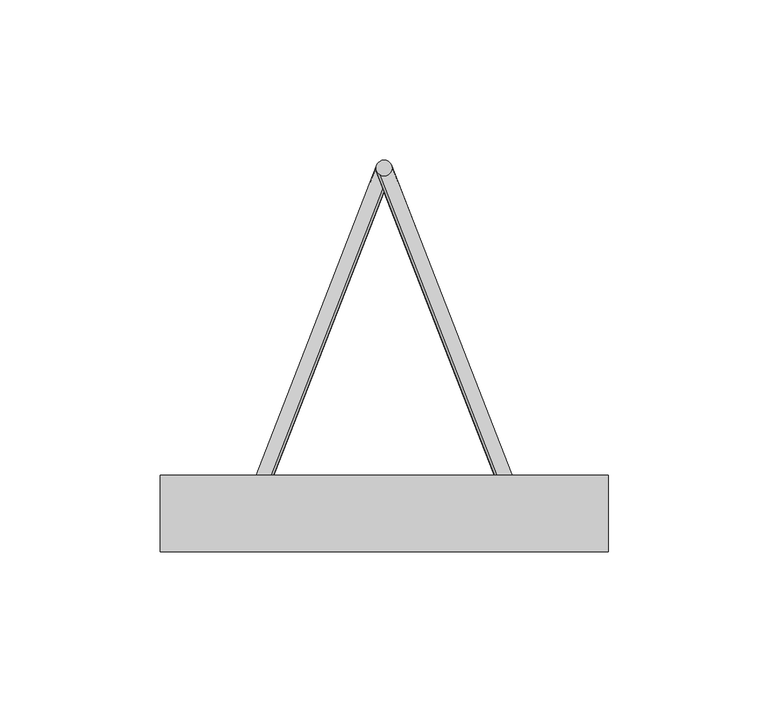
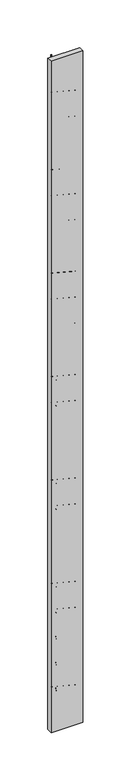
"""IFC4 building model written with IfcOpenShell, lengths in millimetres: proxy geometry, Vigota 7 (Pano 3) (Mf = 137)."""

from ifc_helpers import new_model, si_unit, point, frame, frame_2d, origin, origin_with_axes, origin_2d, place, context, project, spatial, polyline, circle_curve, trimmed, segment, composite_curve, outline, extrude, source, transform, mapped, element, save


def structural_framing_4e036d4d(model_context):
    return source(origin(), model_context, "Body", "SweptSolid", [
        extrude(outline(polyline([(-70.0, 12.0), (70.0, 12.0), (70.0, -12.0), (-70.0, -12.0), (-70.0, 12.0)])), origin_with_axes(), (0.0, 0.0, 1.0), 3115.00107),
        extrude(outline(composite_curve([segment(trimmed(circle_curve(frame_2d((42.0, 0.0)), 2.5), [point((44.5, 0.0))], [point((39.5, 0.0))], False, "CARTESIAN"), True, "CONTINUOUS"), segment(trimmed(circle_curve(frame_2d((42.0, 0.0)), 2.5), [point((39.5, 0.0))], [point((44.5, 0.0))], False, "CARTESIAN"), True, "CONTINUOUS")], self_intersect=False)), frame((0.0, 0.0, 28.0), z_axis=(0.0, 0.0, 1.0), x_axis=(1.0, 0.0, 0.0)), (0.0, 0.0, 1.0), 3059.00107),
        extrude(outline(composite_curve([segment(trimmed(circle_curve(frame_2d((0.0, 108.0)), 2.5), [point((2.5, 108.0))], [point((-2.5, 108.0))], False, "CARTESIAN"), True, "CONTINUOUS"), segment(trimmed(circle_curve(frame_2d((0.0, 108.0)), 2.5), [point((-2.5, 108.0))], [point((2.5, 108.0))], False, "CARTESIAN"), True, "CONTINUOUS")], self_intersect=False)), frame((0.0, 0.0, 67.500535), z_axis=(0.0, 0.0, 1.0), x_axis=(1.0, 0.0, 0.0)), (0.0, 0.0, 1.0), 2980.0),
        extrude(outline(composite_curve([segment(trimmed(circle_curve(origin_2d(), 2.5), [point((2.5, 0.0))], [point((-2.5, 0.0))], False, "CARTESIAN"), True, "CONTINUOUS"), segment(trimmed(circle_curve(origin_2d(), 2.5), [point((-2.5, 0.0))], [point((2.5, 0.0))], False, "CARTESIAN"), True, "CONTINUOUS")], self_intersect=False)), frame((42.0, 0.0, 57.500535), z_axis=(-0.3218603428886276, 0.8276408817707567, 0.4598004898837537), x_axis=(0.8192319205108605, -3.936835275445103e-11, 0.5734623443750141)), (0.0, 0.0, 1.0), 130.491379),
        extrude(outline(composite_curve([segment(trimmed(circle_curve(origin_2d(), 2.5), [point((2.5, 0.0))], [point((-2.5, 0.0))], False, "CARTESIAN"), True, "CONTINUOUS"), segment(trimmed(circle_curve(origin_2d(), 2.5), [point((-2.5, 0.0))], [point((2.5, 0.0))], False, "CARTESIAN"), True, "CONTINUOUS")], self_intersect=False)), frame((0.0, 108.0, 117.500535), z_axis=(0.3218603428886276, -0.8276408817707567, 0.4598004898837537), x_axis=(0.8192319205108605, -3.936835275445103e-11, -0.5734623443750141)), (0.0, 0.0, 1.0), 130.491379),
        extrude(outline(composite_curve([segment(trimmed(circle_curve(origin_2d(), 2.5), [point((2.5, 0.0))], [point((-2.5, 0.0))], False, "CARTESIAN"), True, "CONTINUOUS"), segment(trimmed(circle_curve(origin_2d(), 2.5), [point((-2.5, 0.0))], [point((2.5, 0.0))], False, "CARTESIAN"), True, "CONTINUOUS")], self_intersect=False)), frame((42.0, 0.0, 177.500535), z_axis=(-0.3218603428886276, 0.8276408817707567, 0.4598004898837537), x_axis=(0.8192319205108605, -3.936835275445103e-11, 0.5734623443750141)), (0.0, 0.0, 1.0), 130.491379),
        extrude(outline(composite_curve([segment(trimmed(circle_curve(origin_2d(), 2.5), [point((2.5, 0.0))], [point((-2.5, 0.0))], False, "CARTESIAN"), True, "CONTINUOUS"), segment(trimmed(circle_curve(origin_2d(), 2.5), [point((-2.5, 0.0))], [point((2.5, 0.0))], False, "CARTESIAN"), True, "CONTINUOUS")], self_intersect=False)), frame((0.0, 108.0, 237.500535), z_axis=(0.3218603428886276, -0.8276408817707567, 0.4598004898837537), x_axis=(0.8192319205108605, -3.936835275445103e-11, -0.5734623443750141)), (0.0, 0.0, 1.0), 130.491379),
        extrude(outline(composite_curve([segment(trimmed(circle_curve(origin_2d(), 2.5), [point((2.5, 0.0))], [point((-2.5, 0.0))], False, "CARTESIAN"), True, "CONTINUOUS"), segment(trimmed(circle_curve(origin_2d(), 2.5), [point((-2.5, 0.0))], [point((2.5, 0.0))], False, "CARTESIAN"), True, "CONTINUOUS")], self_intersect=False)), frame((42.0, 0.0, 297.500535), z_axis=(-0.3218603428886276, 0.8276408817707567, 0.4598004898837537), x_axis=(0.8192319205108605, -3.936835275445103e-11, 0.5734623443750141)), (0.0, 0.0, 1.0), 130.491379),
        extrude(outline(composite_curve([segment(trimmed(circle_curve(origin_2d(), 2.5), [point((2.5, 0.0))], [point((-2.5, 0.0))], False, "CARTESIAN"), True, "CONTINUOUS"), segment(trimmed(circle_curve(origin_2d(), 2.5), [point((-2.5, 0.0))], [point((2.5, 0.0))], False, "CARTESIAN"), True, "CONTINUOUS")], self_intersect=False)), frame((0.0, 108.0, 357.500535), z_axis=(0.3218603428886276, -0.8276408817707567, 0.4598004898837537), x_axis=(0.8192319205108605, -3.936835275445103e-11, -0.5734623443750141)), (0.0, 0.0, 1.0), 130.491379),
        extrude(outline(composite_curve([segment(trimmed(circle_curve(origin_2d(), 2.5), [point((2.5, 0.0))], [point((-2.5, 0.0))], False, "CARTESIAN"), True, "CONTINUOUS"), segment(trimmed(circle_curve(origin_2d(), 2.5), [point((-2.5, 0.0))], [point((2.5, 0.0))], False, "CARTESIAN"), True, "CONTINUOUS")], self_intersect=False)), frame((42.0, 0.0, 417.500535), z_axis=(-0.3218603428886276, 0.8276408817707567, 0.4598004898837537), x_axis=(0.8192319205108605, -3.936835275445103e-11, 0.5734623443750141)), (0.0, 0.0, 1.0), 130.491379),
        extrude(outline(composite_curve([segment(trimmed(circle_curve(origin_2d(), 2.5), [point((2.5, 0.0))], [point((-2.5, 0.0))], False, "CARTESIAN"), True, "CONTINUOUS"), segment(trimmed(circle_curve(origin_2d(), 2.5), [point((-2.5, 0.0))], [point((2.5, 0.0))], False, "CARTESIAN"), True, "CONTINUOUS")], self_intersect=False)), frame((0.0, 108.0, 477.500535), z_axis=(0.3218603428886276, -0.8276408817707567, 0.4598004898837537), x_axis=(0.8192319205108605, -3.936835275445103e-11, -0.5734623443750141)), (0.0, 0.0, 1.0), 130.491379),
        extrude(outline(composite_curve([segment(trimmed(circle_curve(origin_2d(), 2.5), [point((2.5, 0.0))], [point((-2.5, 0.0))], False, "CARTESIAN"), True, "CONTINUOUS"), segment(trimmed(circle_curve(origin_2d(), 2.5), [point((-2.5, 0.0))], [point((2.5, 0.0))], False, "CARTESIAN"), True, "CONTINUOUS")], self_intersect=False)), frame((42.0, 0.0, 537.500535), z_axis=(-0.3218603428886276, 0.8276408817707567, 0.4598004898837537), x_axis=(0.8192319205108605, -3.936835275445103e-11, 0.5734623443750141)), (0.0, 0.0, 1.0), 130.491379),
        extrude(outline(composite_curve([segment(trimmed(circle_curve(origin_2d(), 2.5), [point((2.5, 0.0))], [point((-2.5, 0.0))], False, "CARTESIAN"), True, "CONTINUOUS"), segment(trimmed(circle_curve(origin_2d(), 2.5), [point((-2.5, 0.0))], [point((2.5, 0.0))], False, "CARTESIAN"), True, "CONTINUOUS")], self_intersect=False)), frame((0.0, 108.0, 597.500535), z_axis=(0.3218603428886276, -0.8276408817707567, 0.4598004898837537), x_axis=(0.8192319205108605, -3.936835275445103e-11, -0.5734623443750141)), (0.0, 0.0, 1.0), 130.491379),
        extrude(outline(composite_curve([segment(trimmed(circle_curve(origin_2d(), 2.5), [point((2.5, 0.0))], [point((-2.5, 0.0))], False, "CARTESIAN"), True, "CONTINUOUS"), segment(trimmed(circle_curve(origin_2d(), 2.5), [point((-2.5, 0.0))], [point((2.5, 0.0))], False, "CARTESIAN"), True, "CONTINUOUS")], self_intersect=False)), frame((42.0, 0.0, 657.500535), z_axis=(-0.3218603428886276, 0.8276408817707567, 0.4598004898837537), x_axis=(0.8192319205108605, -3.936835275445103e-11, 0.5734623443750141)), (0.0, 0.0, 1.0), 130.491379),
        extrude(outline(composite_curve([segment(trimmed(circle_curve(origin_2d(), 2.5), [point((2.5, 0.0))], [point((-2.5, 0.0))], False, "CARTESIAN"), True, "CONTINUOUS"), segment(trimmed(circle_curve(origin_2d(), 2.5), [point((-2.5, 0.0))], [point((2.5, 0.0))], False, "CARTESIAN"), True, "CONTINUOUS")], self_intersect=False)), frame((0.0, 108.0, 717.500535), z_axis=(0.3218603428886276, -0.8276408817707567, 0.4598004898837537), x_axis=(0.8192319205108605, -3.936835275445103e-11, -0.5734623443750141)), (0.0, 0.0, 1.0), 130.491379),
        extrude(outline(composite_curve([segment(trimmed(circle_curve(origin_2d(), 2.5), [point((2.5, 0.0))], [point((-2.5, 0.0))], False, "CARTESIAN"), True, "CONTINUOUS"), segment(trimmed(circle_curve(origin_2d(), 2.5), [point((-2.5, 0.0))], [point((2.5, 0.0))], False, "CARTESIAN"), True, "CONTINUOUS")], self_intersect=False)), frame((42.0, 0.0, 777.500535), z_axis=(-0.3218603428886276, 0.8276408817707567, 0.4598004898837537), x_axis=(0.8192319205108605, -3.936835275445103e-11, 0.5734623443750141)), (0.0, 0.0, 1.0), 130.491379),
        extrude(outline(composite_curve([segment(trimmed(circle_curve(origin_2d(), 2.5), [point((2.5, 0.0))], [point((-2.5, 0.0))], False, "CARTESIAN"), True, "CONTINUOUS"), segment(trimmed(circle_curve(origin_2d(), 2.5), [point((-2.5, 0.0))], [point((2.5, 0.0))], False, "CARTESIAN"), True, "CONTINUOUS")], self_intersect=False)), frame((0.0, 108.0, 837.500535), z_axis=(0.3218603428886276, -0.8276408817707567, 0.4598004898837537), x_axis=(0.8192319205108605, -3.936835275445103e-11, -0.5734623443750141)), (0.0, 0.0, 1.0), 130.491379),
        extrude(outline(composite_curve([segment(trimmed(circle_curve(origin_2d(), 2.5), [point((2.5, 0.0))], [point((-2.5, 0.0))], False, "CARTESIAN"), True, "CONTINUOUS"), segment(trimmed(circle_curve(origin_2d(), 2.5), [point((-2.5, 0.0))], [point((2.5, 0.0))], False, "CARTESIAN"), True, "CONTINUOUS")], self_intersect=False)), frame((42.0, 0.0, 897.500535), z_axis=(-0.3218603428886276, 0.8276408817707567, 0.4598004898837537), x_axis=(0.8192319205108605, -3.936835275445103e-11, 0.5734623443750141)), (0.0, 0.0, 1.0), 130.491379),
        extrude(outline(composite_curve([segment(trimmed(circle_curve(origin_2d(), 2.5), [point((2.5, 0.0))], [point((-2.5, 0.0))], False, "CARTESIAN"), True, "CONTINUOUS"), segment(trimmed(circle_curve(origin_2d(), 2.5), [point((-2.5, 0.0))], [point((2.5, 0.0))], False, "CARTESIAN"), True, "CONTINUOUS")], self_intersect=False)), frame((0.0, 108.0, 957.500535), z_axis=(0.3218603428886276, -0.8276408817707567, 0.4598004898837537), x_axis=(0.8192319205108605, -3.936835275445103e-11, -0.5734623443750141)), (0.0, 0.0, 1.0), 130.491379),
        extrude(outline(composite_curve([segment(trimmed(circle_curve(origin_2d(), 2.5), [point((2.5, 0.0))], [point((-2.5, 0.0))], False, "CARTESIAN"), True, "CONTINUOUS"), segment(trimmed(circle_curve(origin_2d(), 2.5), [point((-2.5, 0.0))], [point((2.5, 0.0))], False, "CARTESIAN"), True, "CONTINUOUS")], self_intersect=False)), frame((42.0, 0.0, 1017.500535), z_axis=(-0.3218603428886276, 0.8276408817707567, 0.4598004898837537), x_axis=(0.8192319205108605, -3.936835275445103e-11, 0.5734623443750141)), (0.0, 0.0, 1.0), 130.491379),
        extrude(outline(composite_curve([segment(trimmed(circle_curve(origin_2d(), 2.5), [point((2.5, 0.0))], [point((-2.5, 0.0))], False, "CARTESIAN"), True, "CONTINUOUS"), segment(trimmed(circle_curve(origin_2d(), 2.5), [point((-2.5, 0.0))], [point((2.5, 0.0))], False, "CARTESIAN"), True, "CONTINUOUS")], self_intersect=False)), frame((0.0, 108.0, 1077.500535), z_axis=(0.3218603428886276, -0.8276408817707567, 0.4598004898837537), x_axis=(0.8192319205108605, -3.936835275445103e-11, -0.5734623443750141)), (0.0, 0.0, 1.0), 130.491379),
        extrude(outline(composite_curve([segment(trimmed(circle_curve(origin_2d(), 2.5), [point((2.5, 0.0))], [point((-2.5, 0.0))], False, "CARTESIAN"), True, "CONTINUOUS"), segment(trimmed(circle_curve(origin_2d(), 2.5), [point((-2.5, 0.0))], [point((2.5, 0.0))], False, "CARTESIAN"), True, "CONTINUOUS")], self_intersect=False)), frame((42.0, 0.0, 1137.500535), z_axis=(-0.3218603428886276, 0.8276408817707567, 0.4598004898837537), x_axis=(0.8192319205108605, -3.936835275445103e-11, 0.5734623443750141)), (0.0, 0.0, 1.0), 130.491379),
        extrude(outline(composite_curve([segment(trimmed(circle_curve(origin_2d(), 2.5), [point((2.5, 0.0))], [point((-2.5, 0.0))], False, "CARTESIAN"), True, "CONTINUOUS"), segment(trimmed(circle_curve(origin_2d(), 2.5), [point((-2.5, 0.0))], [point((2.5, 0.0))], False, "CARTESIAN"), True, "CONTINUOUS")], self_intersect=False)), frame((0.0, 108.0, 1197.500535), z_axis=(0.3218603428886276, -0.8276408817707567, 0.4598004898837537), x_axis=(0.8192319205108605, -3.936835275445103e-11, -0.5734623443750141)), (0.0, 0.0, 1.0), 130.491379),
        extrude(outline(composite_curve([segment(trimmed(circle_curve(origin_2d(), 2.5), [point((2.5, 0.0))], [point((-2.5, 0.0))], False, "CARTESIAN"), True, "CONTINUOUS"), segment(trimmed(circle_curve(origin_2d(), 2.5), [point((-2.5, 0.0))], [point((2.5, 0.0))], False, "CARTESIAN"), True, "CONTINUOUS")], self_intersect=False)), frame((42.0, 0.0, 1257.500535), z_axis=(-0.3218603428886276, 0.8276408817707567, 0.4598004898837537), x_axis=(0.8192319205108605, -3.936835275445103e-11, 0.5734623443750141)), (0.0, 0.0, 1.0), 130.491379),
        extrude(outline(composite_curve([segment(trimmed(circle_curve(origin_2d(), 2.5), [point((2.5, 0.0))], [point((-2.5, 0.0))], False, "CARTESIAN"), True, "CONTINUOUS"), segment(trimmed(circle_curve(origin_2d(), 2.5), [point((-2.5, 0.0))], [point((2.5, 0.0))], False, "CARTESIAN"), True, "CONTINUOUS")], self_intersect=False)), frame((0.0, 108.0, 1317.500535), z_axis=(0.3218603428886276, -0.8276408817707567, 0.4598004898837537), x_axis=(0.8192319205108605, -3.936835275445103e-11, -0.5734623443750141)), (0.0, 0.0, 1.0), 130.491379),
        extrude(outline(composite_curve([segment(trimmed(circle_curve(origin_2d(), 2.5), [point((2.5, 0.0))], [point((-2.5, 0.0))], False, "CARTESIAN"), True, "CONTINUOUS"), segment(trimmed(circle_curve(origin_2d(), 2.5), [point((-2.5, 0.0))], [point((2.5, 0.0))], False, "CARTESIAN"), True, "CONTINUOUS")], self_intersect=False)), frame((42.0, 0.0, 1377.500535), z_axis=(-0.3218603428886276, 0.8276408817707567, 0.4598004898837537), x_axis=(0.8192319205108605, -3.936835275445103e-11, 0.5734623443750141)), (0.0, 0.0, 1.0), 130.491379),
        extrude(outline(composite_curve([segment(trimmed(circle_curve(origin_2d(), 2.5), [point((2.5, 0.0))], [point((-2.5, 0.0))], False, "CARTESIAN"), True, "CONTINUOUS"), segment(trimmed(circle_curve(origin_2d(), 2.5), [point((-2.5, 0.0))], [point((2.5, 0.0))], False, "CARTESIAN"), True, "CONTINUOUS")], self_intersect=False)), frame((0.0, 108.0, 1437.500535), z_axis=(0.3218603428886276, -0.8276408817707567, 0.4598004898837537), x_axis=(0.8192319205108605, -3.936835275445103e-11, -0.5734623443750141)), (0.0, 0.0, 1.0), 130.491379),
        extrude(outline(composite_curve([segment(trimmed(circle_curve(origin_2d(), 2.5), [point((2.5, 0.0))], [point((-2.5, 0.0))], False, "CARTESIAN"), True, "CONTINUOUS"), segment(trimmed(circle_curve(origin_2d(), 2.5), [point((-2.5, 0.0))], [point((2.5, 0.0))], False, "CARTESIAN"), True, "CONTINUOUS")], self_intersect=False)), frame((42.0, 0.0, 1497.500535), z_axis=(-0.3218603428886276, 0.8276408817707567, 0.4598004898837537), x_axis=(0.8192319205108605, -3.936835275445103e-11, 0.5734623443750141)), (0.0, 0.0, 1.0), 130.491379),
        extrude(outline(composite_curve([segment(trimmed(circle_curve(origin_2d(), 2.5), [point((2.5, 0.0))], [point((-2.5, 0.0))], False, "CARTESIAN"), True, "CONTINUOUS"), segment(trimmed(circle_curve(origin_2d(), 2.5), [point((-2.5, 0.0))], [point((2.5, 0.0))], False, "CARTESIAN"), True, "CONTINUOUS")], self_intersect=False)), frame((0.0, 108.0, 1557.500535), z_axis=(0.3218603428886276, -0.8276408817707567, 0.4598004898837537), x_axis=(0.8192319205108605, -3.936835275445103e-11, -0.5734623443750141)), (0.0, 0.0, 1.0), 130.491379),
        extrude(outline(composite_curve([segment(trimmed(circle_curve(origin_2d(), 2.5), [point((2.5, 0.0))], [point((-2.5, 0.0))], False, "CARTESIAN"), True, "CONTINUOUS"), segment(trimmed(circle_curve(origin_2d(), 2.5), [point((-2.5, 0.0))], [point((2.5, 0.0))], False, "CARTESIAN"), True, "CONTINUOUS")], self_intersect=False)), frame((42.0, 0.0, 1617.500535), z_axis=(-0.3218603428886276, 0.8276408817707567, 0.4598004898837537), x_axis=(0.8192319205108605, -3.936835275445103e-11, 0.5734623443750141)), (0.0, 0.0, 1.0), 130.491379),
        extrude(outline(composite_curve([segment(trimmed(circle_curve(origin_2d(), 2.5), [point((2.5, 0.0))], [point((-2.5, 0.0))], False, "CARTESIAN"), True, "CONTINUOUS"), segment(trimmed(circle_curve(origin_2d(), 2.5), [point((-2.5, 0.0))], [point((2.5, 0.0))], False, "CARTESIAN"), True, "CONTINUOUS")], self_intersect=False)), frame((0.0, 108.0, 1677.500535), z_axis=(0.3218603428886276, -0.8276408817707567, 0.4598004898837537), x_axis=(0.8192319205108605, -3.936835275445103e-11, -0.5734623443750141)), (0.0, 0.0, 1.0), 130.491379),
        extrude(outline(composite_curve([segment(trimmed(circle_curve(origin_2d(), 2.5), [point((2.5, 0.0))], [point((-2.5, 0.0))], False, "CARTESIAN"), True, "CONTINUOUS"), segment(trimmed(circle_curve(origin_2d(), 2.5), [point((-2.5, 0.0))], [point((2.5, 0.0))], False, "CARTESIAN"), True, "CONTINUOUS")], self_intersect=False)), frame((42.0, 0.0, 1737.500535), z_axis=(-0.3218603428886276, 0.8276408817707567, 0.4598004898837537), x_axis=(0.8192319205108605, -3.936835275445103e-11, 0.5734623443750141)), (0.0, 0.0, 1.0), 130.491379),
        extrude(outline(composite_curve([segment(trimmed(circle_curve(origin_2d(), 2.5), [point((2.5, 0.0))], [point((-2.5, 0.0))], False, "CARTESIAN"), True, "CONTINUOUS"), segment(trimmed(circle_curve(origin_2d(), 2.5), [point((-2.5, 0.0))], [point((2.5, 0.0))], False, "CARTESIAN"), True, "CONTINUOUS")], self_intersect=False)), frame((0.0, 108.0, 1797.500535), z_axis=(0.3218603428886276, -0.8276408817707567, 0.4598004898837537), x_axis=(0.8192319205108605, -3.936835275445103e-11, -0.5734623443750141)), (0.0, 0.0, 1.0), 130.491379),
        extrude(outline(composite_curve([segment(trimmed(circle_curve(origin_2d(), 2.5), [point((2.5, 0.0))], [point((-2.5, 0.0))], False, "CARTESIAN"), True, "CONTINUOUS"), segment(trimmed(circle_curve(origin_2d(), 2.5), [point((-2.5, 0.0))], [point((2.5, 0.0))], False, "CARTESIAN"), True, "CONTINUOUS")], self_intersect=False)), frame((42.0, 0.0, 1857.500535), z_axis=(-0.3218603428886276, 0.8276408817707567, 0.4598004898837537), x_axis=(0.8192319205108605, -3.936835275445103e-11, 0.5734623443750141)), (0.0, 0.0, 1.0), 130.491379),
        extrude(outline(composite_curve([segment(trimmed(circle_curve(origin_2d(), 2.5), [point((2.5, 0.0))], [point((-2.5, 0.0))], False, "CARTESIAN"), True, "CONTINUOUS"), segment(trimmed(circle_curve(origin_2d(), 2.5), [point((-2.5, 0.0))], [point((2.5, 0.0))], False, "CARTESIAN"), True, "CONTINUOUS")], self_intersect=False)), frame((0.0, 108.0, 1917.500535), z_axis=(0.3218603428886276, -0.8276408817707567, 0.4598004898837537), x_axis=(0.8192319205108605, -3.936835275445103e-11, -0.5734623443750141)), (0.0, 0.0, 1.0), 130.491379),
        extrude(outline(composite_curve([segment(trimmed(circle_curve(origin_2d(), 2.5), [point((2.5, 0.0))], [point((-2.5, 0.0))], False, "CARTESIAN"), True, "CONTINUOUS"), segment(trimmed(circle_curve(origin_2d(), 2.5), [point((-2.5, 0.0))], [point((2.5, 0.0))], False, "CARTESIAN"), True, "CONTINUOUS")], self_intersect=False)), frame((42.0, 0.0, 1977.500535), z_axis=(-0.3218603428886276, 0.8276408817707567, 0.4598004898837537), x_axis=(0.8192319205108605, -3.936835275445103e-11, 0.5734623443750141)), (0.0, 0.0, 1.0), 130.491379),
        extrude(outline(composite_curve([segment(trimmed(circle_curve(origin_2d(), 2.5), [point((2.5, 0.0))], [point((-2.5, 0.0))], False, "CARTESIAN"), True, "CONTINUOUS"), segment(trimmed(circle_curve(origin_2d(), 2.5), [point((-2.5, 0.0))], [point((2.5, 0.0))], False, "CARTESIAN"), True, "CONTINUOUS")], self_intersect=False)), frame((0.0, 108.0, 2037.500535), z_axis=(0.3218603428886276, -0.8276408817707567, 0.4598004898837537), x_axis=(0.8192319205108605, -3.936835275445103e-11, -0.5734623443750141)), (0.0, 0.0, 1.0), 130.491379),
        extrude(outline(composite_curve([segment(trimmed(circle_curve(origin_2d(), 2.5), [point((2.5, 0.0))], [point((-2.5, 0.0))], False, "CARTESIAN"), True, "CONTINUOUS"), segment(trimmed(circle_curve(origin_2d(), 2.5), [point((-2.5, 0.0))], [point((2.5, 0.0))], False, "CARTESIAN"), True, "CONTINUOUS")], self_intersect=False)), frame((42.0, 0.0, 2097.500535), z_axis=(-0.3218603428886276, 0.8276408817707567, 0.4598004898837537), x_axis=(0.8192319205108605, -3.936835275445103e-11, 0.5734623443750141)), (0.0, 0.0, 1.0), 130.491379),
        extrude(outline(composite_curve([segment(trimmed(circle_curve(origin_2d(), 2.5), [point((2.5, 0.0))], [point((-2.5, 0.0))], False, "CARTESIAN"), True, "CONTINUOUS"), segment(trimmed(circle_curve(origin_2d(), 2.5), [point((-2.5, 0.0))], [point((2.5, 0.0))], False, "CARTESIAN"), True, "CONTINUOUS")], self_intersect=False)), frame((0.0, 108.0, 2157.500535), z_axis=(0.3218603428886276, -0.8276408817707567, 0.4598004898837537), x_axis=(0.8192319205108605, -3.936835275445103e-11, -0.5734623443750141)), (0.0, 0.0, 1.0), 130.491379),
        extrude(outline(composite_curve([segment(trimmed(circle_curve(origin_2d(), 2.5), [point((2.5, 0.0))], [point((-2.5, 0.0))], False, "CARTESIAN"), True, "CONTINUOUS"), segment(trimmed(circle_curve(origin_2d(), 2.5), [point((-2.5, 0.0))], [point((2.5, 0.0))], False, "CARTESIAN"), True, "CONTINUOUS")], self_intersect=False)), frame((42.0, 0.0, 2217.500535), z_axis=(-0.3218603428886276, 0.8276408817707567, 0.4598004898837537), x_axis=(0.8192319205108605, -3.936835275445103e-11, 0.5734623443750141)), (0.0, 0.0, 1.0), 130.491379),
        extrude(outline(composite_curve([segment(trimmed(circle_curve(origin_2d(), 2.5), [point((2.5, 0.0))], [point((-2.5, 0.0))], False, "CARTESIAN"), True, "CONTINUOUS"), segment(trimmed(circle_curve(origin_2d(), 2.5), [point((-2.5, 0.0))], [point((2.5, 0.0))], False, "CARTESIAN"), True, "CONTINUOUS")], self_intersect=False)), frame((0.0, 108.0, 2277.500535), z_axis=(0.3218603428886276, -0.8276408817707567, 0.4598004898837537), x_axis=(0.8192319205108605, -3.936835275445103e-11, -0.5734623443750141)), (0.0, 0.0, 1.0), 130.491379),
        extrude(outline(composite_curve([segment(trimmed(circle_curve(origin_2d(), 2.5), [point((2.5, 0.0))], [point((-2.5, 0.0))], False, "CARTESIAN"), True, "CONTINUOUS"), segment(trimmed(circle_curve(origin_2d(), 2.5), [point((-2.5, 0.0))], [point((2.5, 0.0))], False, "CARTESIAN"), True, "CONTINUOUS")], self_intersect=False)), frame((42.0, 0.0, 2337.500535), z_axis=(-0.3218603428886276, 0.8276408817707567, 0.4598004898837537), x_axis=(0.8192319205108605, -3.936835275445103e-11, 0.5734623443750141)), (0.0, 0.0, 1.0), 130.491379),
        extrude(outline(composite_curve([segment(trimmed(circle_curve(origin_2d(), 2.5), [point((2.5, 0.0))], [point((-2.5, 0.0))], False, "CARTESIAN"), True, "CONTINUOUS"), segment(trimmed(circle_curve(origin_2d(), 2.5), [point((-2.5, 0.0))], [point((2.5, 0.0))], False, "CARTESIAN"), True, "CONTINUOUS")], self_intersect=False)), frame((0.0, 108.0, 2397.500535), z_axis=(0.3218603428886276, -0.8276408817707567, 0.4598004898837537), x_axis=(0.8192319205108605, -3.936835275445103e-11, -0.5734623443750141)), (0.0, 0.0, 1.0), 130.491379),
        extrude(outline(composite_curve([segment(trimmed(circle_curve(origin_2d(), 2.5), [point((2.5, 0.0))], [point((-2.5, 0.0))], False, "CARTESIAN"), True, "CONTINUOUS"), segment(trimmed(circle_curve(origin_2d(), 2.5), [point((-2.5, 0.0))], [point((2.5, 0.0))], False, "CARTESIAN"), True, "CONTINUOUS")], self_intersect=False)), frame((42.0, 0.0, 2457.500535), z_axis=(-0.3218603428886276, 0.8276408817707567, 0.4598004898837537), x_axis=(0.8192319205108605, -3.936835275445103e-11, 0.5734623443750141)), (0.0, 0.0, 1.0), 130.491379),
        extrude(outline(composite_curve([segment(trimmed(circle_curve(origin_2d(), 2.5), [point((2.5, 0.0))], [point((-2.5, 0.0))], False, "CARTESIAN"), True, "CONTINUOUS"), segment(trimmed(circle_curve(origin_2d(), 2.5), [point((-2.5, 0.0))], [point((2.5, 0.0))], False, "CARTESIAN"), True, "CONTINUOUS")], self_intersect=False)), frame((0.0, 108.0, 2517.500535), z_axis=(0.3218603428886276, -0.8276408817707567, 0.4598004898837537), x_axis=(0.8192319205108605, -3.936835275445103e-11, -0.5734623443750141)), (0.0, 0.0, 1.0), 130.491379),
        extrude(outline(composite_curve([segment(trimmed(circle_curve(origin_2d(), 2.5), [point((2.5, 0.0))], [point((-2.5, 0.0))], False, "CARTESIAN"), True, "CONTINUOUS"), segment(trimmed(circle_curve(origin_2d(), 2.5), [point((-2.5, 0.0))], [point((2.5, 0.0))], False, "CARTESIAN"), True, "CONTINUOUS")], self_intersect=False)), frame((42.0, 0.0, 2577.500535), z_axis=(-0.3218603428886276, 0.8276408817707567, 0.4598004898837537), x_axis=(0.8192319205108605, -3.936835275445103e-11, 0.5734623443750141)), (0.0, 0.0, 1.0), 130.491379),
        extrude(outline(composite_curve([segment(trimmed(circle_curve(origin_2d(), 2.5), [point((2.5, 0.0))], [point((-2.5, 0.0))], False, "CARTESIAN"), True, "CONTINUOUS"), segment(trimmed(circle_curve(origin_2d(), 2.5), [point((-2.5, 0.0))], [point((2.5, 0.0))], False, "CARTESIAN"), True, "CONTINUOUS")], self_intersect=False)), frame((0.0, 108.0, 2637.500535), z_axis=(0.3218603428886276, -0.8276408817707567, 0.4598004898837537), x_axis=(0.8192319205108605, -3.936835275445103e-11, -0.5734623443750141)), (0.0, 0.0, 1.0), 130.491379),
        extrude(outline(composite_curve([segment(trimmed(circle_curve(origin_2d(), 2.5), [point((2.5, 0.0))], [point((-2.5, 0.0))], False, "CARTESIAN"), True, "CONTINUOUS"), segment(trimmed(circle_curve(origin_2d(), 2.5), [point((-2.5, 0.0))], [point((2.5, 0.0))], False, "CARTESIAN"), True, "CONTINUOUS")], self_intersect=False)), frame((42.0, 0.0, 2697.500535), z_axis=(-0.3218603428886276, 0.8276408817707567, 0.4598004898837537), x_axis=(0.8192319205108605, -3.936835275445103e-11, 0.5734623443750141)), (0.0, 0.0, 1.0), 130.491379),
        extrude(outline(composite_curve([segment(trimmed(circle_curve(origin_2d(), 2.5), [point((2.5, 0.0))], [point((-2.5, 0.0))], False, "CARTESIAN"), True, "CONTINUOUS"), segment(trimmed(circle_curve(origin_2d(), 2.5), [point((-2.5, 0.0))], [point((2.5, 0.0))], False, "CARTESIAN"), True, "CONTINUOUS")], self_intersect=False)), frame((0.0, 108.0, 2757.500535), z_axis=(0.3218603428886276, -0.8276408817707567, 0.4598004898837537), x_axis=(0.8192319205108605, -3.936835275445103e-11, -0.5734623443750141)), (0.0, 0.0, 1.0), 130.491379),
        extrude(outline(composite_curve([segment(trimmed(circle_curve(origin_2d(), 2.5), [point((2.5, 0.0))], [point((-2.5, 0.0))], False, "CARTESIAN"), True, "CONTINUOUS"), segment(trimmed(circle_curve(origin_2d(), 2.5), [point((-2.5, 0.0))], [point((2.5, 0.0))], False, "CARTESIAN"), True, "CONTINUOUS")], self_intersect=False)), frame((42.0, 0.0, 2817.500535), z_axis=(-0.3218603428886276, 0.8276408817707567, 0.4598004898837537), x_axis=(0.8192319205108605, -3.936835275445103e-11, 0.5734623443750141)), (0.0, 0.0, 1.0), 130.491379),
        extrude(outline(composite_curve([segment(trimmed(circle_curve(origin_2d(), 2.5), [point((2.5, 0.0))], [point((-2.5, 0.0))], False, "CARTESIAN"), True, "CONTINUOUS"), segment(trimmed(circle_curve(origin_2d(), 2.5), [point((-2.5, 0.0))], [point((2.5, 0.0))], False, "CARTESIAN"), True, "CONTINUOUS")], self_intersect=False)), frame((0.0, 108.0, 2877.500535), z_axis=(0.3218603428886276, -0.8276408817707567, 0.4598004898837537), x_axis=(0.8192319205108605, -3.936835275445103e-11, -0.5734623443750141)), (0.0, 0.0, 1.0), 130.491379),
        extrude(outline(composite_curve([segment(trimmed(circle_curve(origin_2d(), 2.5), [point((2.5, 0.0))], [point((-2.5, 0.0))], False, "CARTESIAN"), True, "CONTINUOUS"), segment(trimmed(circle_curve(origin_2d(), 2.5), [point((-2.5, 0.0))], [point((2.5, 0.0))], False, "CARTESIAN"), True, "CONTINUOUS")], self_intersect=False)), frame((42.0, 0.0, 2937.500535), z_axis=(-0.3218603428886276, 0.8276408817707567, 0.4598004898837537), x_axis=(0.8192319205108605, -3.936835275445103e-11, 0.5734623443750141)), (0.0, 0.0, 1.0), 130.491379),
        extrude(outline(composite_curve([segment(trimmed(circle_curve(origin_2d(), 2.5), [point((2.5, 0.0))], [point((-2.5, 0.0))], False, "CARTESIAN"), True, "CONTINUOUS"), segment(trimmed(circle_curve(origin_2d(), 2.5), [point((-2.5, 0.0))], [point((2.5, 0.0))], False, "CARTESIAN"), True, "CONTINUOUS")], self_intersect=False)), frame((0.0, 108.0, 2997.500535), z_axis=(0.3218603428886276, -0.8276408817707567, 0.4598004898837537), x_axis=(0.8192319205108605, -3.936835275445103e-11, -0.5734623443750141)), (0.0, 0.0, 1.0), 130.491379),
        extrude(outline(composite_curve([segment(trimmed(circle_curve(frame_2d((-42.0, 0.0)), 2.5), [point((-39.5, 0.0))], [point((-44.5, 0.0))], False, "CARTESIAN"), True, "CONTINUOUS"), segment(trimmed(circle_curve(frame_2d((-42.0, 0.0)), 2.5), [point((-44.5, 0.0))], [point((-39.5, 0.0))], False, "CARTESIAN"), True, "CONTINUOUS")], self_intersect=False)), frame((0.0, 0.0, 28.0), z_axis=(0.0, 0.0, 1.0), x_axis=(1.0, 0.0, 0.0)), (0.0, 0.0, 1.0), 3059.00107),
        extrude(outline(composite_curve([segment(trimmed(circle_curve(origin_2d(), 2.5), [point((2.5, 0.0))], [point((-2.5, 0.0))], False, "CARTESIAN"), True, "CONTINUOUS"), segment(trimmed(circle_curve(origin_2d(), 2.5), [point((-2.5, 0.0))], [point((2.5, 0.0))], False, "CARTESIAN"), True, "CONTINUOUS")], self_intersect=False)), frame((-42.0, 0.0, 57.500535), z_axis=(0.3218603428886276, 0.8276408817707567, 0.4598004898837537), x_axis=(0.8192319205108605, 3.936835275445103e-11, -0.5734623443750141)), (0.0, 0.0, 1.0), 130.491379),
        extrude(outline(composite_curve([segment(trimmed(circle_curve(origin_2d(), 2.5), [point((2.5, 0.0))], [point((-2.5, 0.0))], False, "CARTESIAN"), True, "CONTINUOUS"), segment(trimmed(circle_curve(origin_2d(), 2.5), [point((-2.5, 0.0))], [point((2.5, 0.0))], False, "CARTESIAN"), True, "CONTINUOUS")], self_intersect=False)), frame((0.0, 108.0, 117.500535), z_axis=(-0.3218603428886276, -0.8276408817707567, 0.4598004898837537), x_axis=(0.8192319205108605, 3.936835275445103e-11, 0.5734623443750141)), (0.0, 0.0, 1.0), 130.491379),
        extrude(outline(composite_curve([segment(trimmed(circle_curve(origin_2d(), 2.5), [point((2.5, 0.0))], [point((-2.5, 0.0))], False, "CARTESIAN"), True, "CONTINUOUS"), segment(trimmed(circle_curve(origin_2d(), 2.5), [point((-2.5, 0.0))], [point((2.5, 0.0))], False, "CARTESIAN"), True, "CONTINUOUS")], self_intersect=False)), frame((-42.0, 0.0, 177.500535), z_axis=(0.3218603428886276, 0.8276408817707567, 0.4598004898837537), x_axis=(0.8192319205108605, 3.936835275445103e-11, -0.5734623443750141)), (0.0, 0.0, 1.0), 130.491379),
        extrude(outline(composite_curve([segment(trimmed(circle_curve(origin_2d(), 2.5), [point((2.5, 0.0))], [point((-2.5, 0.0))], False, "CARTESIAN"), True, "CONTINUOUS"), segment(trimmed(circle_curve(origin_2d(), 2.5), [point((-2.5, 0.0))], [point((2.5, 0.0))], False, "CARTESIAN"), True, "CONTINUOUS")], self_intersect=False)), frame((0.0, 108.0, 237.500535), z_axis=(-0.3218603428886276, -0.8276408817707567, 0.4598004898837537), x_axis=(0.8192319205108605, 3.936835275445103e-11, 0.5734623443750141)), (0.0, 0.0, 1.0), 130.491379),
        extrude(outline(composite_curve([segment(trimmed(circle_curve(origin_2d(), 2.5), [point((2.5, 0.0))], [point((-2.5, 0.0))], False, "CARTESIAN"), True, "CONTINUOUS"), segment(trimmed(circle_curve(origin_2d(), 2.5), [point((-2.5, 0.0))], [point((2.5, 0.0))], False, "CARTESIAN"), True, "CONTINUOUS")], self_intersect=False)), frame((-42.0, 0.0, 297.500535), z_axis=(0.3218603428886276, 0.8276408817707567, 0.4598004898837537), x_axis=(0.8192319205108605, 3.936835275445103e-11, -0.5734623443750141)), (0.0, 0.0, 1.0), 130.491379),
        extrude(outline(composite_curve([segment(trimmed(circle_curve(origin_2d(), 2.5), [point((2.5, 0.0))], [point((-2.5, 0.0))], False, "CARTESIAN"), True, "CONTINUOUS"), segment(trimmed(circle_curve(origin_2d(), 2.5), [point((-2.5, 0.0))], [point((2.5, 0.0))], False, "CARTESIAN"), True, "CONTINUOUS")], self_intersect=False)), frame((0.0, 108.0, 357.500535), z_axis=(-0.3218603428886276, -0.8276408817707567, 0.4598004898837537), x_axis=(0.8192319205108605, 3.936835275445103e-11, 0.5734623443750141)), (0.0, 0.0, 1.0), 130.491379),
        extrude(outline(composite_curve([segment(trimmed(circle_curve(origin_2d(), 2.5), [point((2.5, 0.0))], [point((-2.5, 0.0))], False, "CARTESIAN"), True, "CONTINUOUS"), segment(trimmed(circle_curve(origin_2d(), 2.5), [point((-2.5, 0.0))], [point((2.5, 0.0))], False, "CARTESIAN"), True, "CONTINUOUS")], self_intersect=False)), frame((-42.0, 0.0, 417.500535), z_axis=(0.3218603428886276, 0.8276408817707567, 0.4598004898837537), x_axis=(0.8192319205108605, 3.936835275445103e-11, -0.5734623443750141)), (0.0, 0.0, 1.0), 130.491379),
        extrude(outline(composite_curve([segment(trimmed(circle_curve(origin_2d(), 2.5), [point((2.5, 0.0))], [point((-2.5, 0.0))], False, "CARTESIAN"), True, "CONTINUOUS"), segment(trimmed(circle_curve(origin_2d(), 2.5), [point((-2.5, 0.0))], [point((2.5, 0.0))], False, "CARTESIAN"), True, "CONTINUOUS")], self_intersect=False)), frame((0.0, 108.0, 477.500535), z_axis=(-0.3218603428886276, -0.8276408817707567, 0.4598004898837537), x_axis=(0.8192319205108605, 3.936835275445103e-11, 0.5734623443750141)), (0.0, 0.0, 1.0), 130.491379),
        extrude(outline(composite_curve([segment(trimmed(circle_curve(origin_2d(), 2.5), [point((2.5, 0.0))], [point((-2.5, 0.0))], False, "CARTESIAN"), True, "CONTINUOUS"), segment(trimmed(circle_curve(origin_2d(), 2.5), [point((-2.5, 0.0))], [point((2.5, 0.0))], False, "CARTESIAN"), True, "CONTINUOUS")], self_intersect=False)), frame((-42.0, 0.0, 537.500535), z_axis=(0.3218603428886276, 0.8276408817707567, 0.4598004898837537), x_axis=(0.8192319205108605, 3.936835275445103e-11, -0.5734623443750141)), (0.0, 0.0, 1.0), 130.491379),
        extrude(outline(composite_curve([segment(trimmed(circle_curve(origin_2d(), 2.5), [point((2.5, 0.0))], [point((-2.5, 0.0))], False, "CARTESIAN"), True, "CONTINUOUS"), segment(trimmed(circle_curve(origin_2d(), 2.5), [point((-2.5, 0.0))], [point((2.5, 0.0))], False, "CARTESIAN"), True, "CONTINUOUS")], self_intersect=False)), frame((0.0, 108.0, 597.500535), z_axis=(-0.3218603428886276, -0.8276408817707567, 0.4598004898837537), x_axis=(0.8192319205108605, 3.936835275445103e-11, 0.5734623443750141)), (0.0, 0.0, 1.0), 130.491379),
        extrude(outline(composite_curve([segment(trimmed(circle_curve(origin_2d(), 2.5), [point((2.5, 0.0))], [point((-2.5, 0.0))], False, "CARTESIAN"), True, "CONTINUOUS"), segment(trimmed(circle_curve(origin_2d(), 2.5), [point((-2.5, 0.0))], [point((2.5, 0.0))], False, "CARTESIAN"), True, "CONTINUOUS")], self_intersect=False)), frame((-42.0, 0.0, 657.500535), z_axis=(0.3218603428886276, 0.8276408817707567, 0.4598004898837537), x_axis=(0.8192319205108605, 3.936835275445103e-11, -0.5734623443750141)), (0.0, 0.0, 1.0), 130.491379),
        extrude(outline(composite_curve([segment(trimmed(circle_curve(origin_2d(), 2.5), [point((2.5, 0.0))], [point((-2.5, 0.0))], False, "CARTESIAN"), True, "CONTINUOUS"), segment(trimmed(circle_curve(origin_2d(), 2.5), [point((-2.5, 0.0))], [point((2.5, 0.0))], False, "CARTESIAN"), True, "CONTINUOUS")], self_intersect=False)), frame((0.0, 108.0, 717.500535), z_axis=(-0.3218603428886276, -0.8276408817707567, 0.4598004898837537), x_axis=(0.8192319205108605, 3.936835275445103e-11, 0.5734623443750141)), (0.0, 0.0, 1.0), 130.491379),
        extrude(outline(composite_curve([segment(trimmed(circle_curve(origin_2d(), 2.5), [point((2.5, 0.0))], [point((-2.5, 0.0))], False, "CARTESIAN"), True, "CONTINUOUS"), segment(trimmed(circle_curve(origin_2d(), 2.5), [point((-2.5, 0.0))], [point((2.5, 0.0))], False, "CARTESIAN"), True, "CONTINUOUS")], self_intersect=False)), frame((-42.0, 0.0, 777.500535), z_axis=(0.3218603428886276, 0.8276408817707567, 0.4598004898837537), x_axis=(0.8192319205108605, 3.936835275445103e-11, -0.5734623443750141)), (0.0, 0.0, 1.0), 130.491379),
        extrude(outline(composite_curve([segment(trimmed(circle_curve(origin_2d(), 2.5), [point((2.5, 0.0))], [point((-2.5, 0.0))], False, "CARTESIAN"), True, "CONTINUOUS"), segment(trimmed(circle_curve(origin_2d(), 2.5), [point((-2.5, 0.0))], [point((2.5, 0.0))], False, "CARTESIAN"), True, "CONTINUOUS")], self_intersect=False)), frame((0.0, 108.0, 837.500535), z_axis=(-0.3218603428886276, -0.8276408817707567, 0.4598004898837537), x_axis=(0.8192319205108605, 3.936835275445103e-11, 0.5734623443750141)), (0.0, 0.0, 1.0), 130.491379),
        extrude(outline(composite_curve([segment(trimmed(circle_curve(origin_2d(), 2.5), [point((2.5, 0.0))], [point((-2.5, 0.0))], False, "CARTESIAN"), True, "CONTINUOUS"), segment(trimmed(circle_curve(origin_2d(), 2.5), [point((-2.5, 0.0))], [point((2.5, 0.0))], False, "CARTESIAN"), True, "CONTINUOUS")], self_intersect=False)), frame((-42.0, 0.0, 897.500535), z_axis=(0.3218603428886276, 0.8276408817707567, 0.4598004898837537), x_axis=(0.8192319205108605, 3.936835275445103e-11, -0.5734623443750141)), (0.0, 0.0, 1.0), 130.491379),
        extrude(outline(composite_curve([segment(trimmed(circle_curve(origin_2d(), 2.5), [point((2.5, 0.0))], [point((-2.5, 0.0))], False, "CARTESIAN"), True, "CONTINUOUS"), segment(trimmed(circle_curve(origin_2d(), 2.5), [point((-2.5, 0.0))], [point((2.5, 0.0))], False, "CARTESIAN"), True, "CONTINUOUS")], self_intersect=False)), frame((0.0, 108.0, 957.500535), z_axis=(-0.3218603428886276, -0.8276408817707567, 0.4598004898837537), x_axis=(0.8192319205108605, 3.936835275445103e-11, 0.5734623443750141)), (0.0, 0.0, 1.0), 130.491379),
        extrude(outline(composite_curve([segment(trimmed(circle_curve(origin_2d(), 2.5), [point((2.5, 0.0))], [point((-2.5, 0.0))], False, "CARTESIAN"), True, "CONTINUOUS"), segment(trimmed(circle_curve(origin_2d(), 2.5), [point((-2.5, 0.0))], [point((2.5, 0.0))], False, "CARTESIAN"), True, "CONTINUOUS")], self_intersect=False)), frame((-42.0, 0.0, 1017.500535), z_axis=(0.3218603428886276, 0.8276408817707567, 0.4598004898837537), x_axis=(0.8192319205108605, 3.936835275445103e-11, -0.5734623443750141)), (0.0, 0.0, 1.0), 130.491379),
        extrude(outline(composite_curve([segment(trimmed(circle_curve(origin_2d(), 2.5), [point((2.5, 0.0))], [point((-2.5, 0.0))], False, "CARTESIAN"), True, "CONTINUOUS"), segment(trimmed(circle_curve(origin_2d(), 2.5), [point((-2.5, 0.0))], [point((2.5, 0.0))], False, "CARTESIAN"), True, "CONTINUOUS")], self_intersect=False)), frame((0.0, 108.0, 1077.500535), z_axis=(-0.3218603428886276, -0.8276408817707567, 0.4598004898837537), x_axis=(0.8192319205108605, 3.936835275445103e-11, 0.5734623443750141)), (0.0, 0.0, 1.0), 130.491379),
        extrude(outline(composite_curve([segment(trimmed(circle_curve(origin_2d(), 2.5), [point((2.5, 0.0))], [point((-2.5, 0.0))], False, "CARTESIAN"), True, "CONTINUOUS"), segment(trimmed(circle_curve(origin_2d(), 2.5), [point((-2.5, 0.0))], [point((2.5, 0.0))], False, "CARTESIAN"), True, "CONTINUOUS")], self_intersect=False)), frame((-42.0, 0.0, 1137.500535), z_axis=(0.3218603428886276, 0.8276408817707567, 0.4598004898837537), x_axis=(0.8192319205108605, 3.936835275445103e-11, -0.5734623443750141)), (0.0, 0.0, 1.0), 130.491379),
        extrude(outline(composite_curve([segment(trimmed(circle_curve(origin_2d(), 2.5), [point((2.5, 0.0))], [point((-2.5, 0.0))], False, "CARTESIAN"), True, "CONTINUOUS"), segment(trimmed(circle_curve(origin_2d(), 2.5), [point((-2.5, 0.0))], [point((2.5, 0.0))], False, "CARTESIAN"), True, "CONTINUOUS")], self_intersect=False)), frame((0.0, 108.0, 1197.500535), z_axis=(-0.3218603428886276, -0.8276408817707567, 0.4598004898837537), x_axis=(0.8192319205108605, 3.936835275445103e-11, 0.5734623443750141)), (0.0, 0.0, 1.0), 130.491379),
        extrude(outline(composite_curve([segment(trimmed(circle_curve(origin_2d(), 2.5), [point((2.5, 0.0))], [point((-2.5, 0.0))], False, "CARTESIAN"), True, "CONTINUOUS"), segment(trimmed(circle_curve(origin_2d(), 2.5), [point((-2.5, 0.0))], [point((2.5, 0.0))], False, "CARTESIAN"), True, "CONTINUOUS")], self_intersect=False)), frame((-42.0, 0.0, 1257.500535), z_axis=(0.3218603428886276, 0.8276408817707567, 0.4598004898837537), x_axis=(0.8192319205108605, 3.936835275445103e-11, -0.5734623443750141)), (0.0, 0.0, 1.0), 130.491379),
        extrude(outline(composite_curve([segment(trimmed(circle_curve(origin_2d(), 2.5), [point((2.5, 0.0))], [point((-2.5, 0.0))], False, "CARTESIAN"), True, "CONTINUOUS"), segment(trimmed(circle_curve(origin_2d(), 2.5), [point((-2.5, 0.0))], [point((2.5, 0.0))], False, "CARTESIAN"), True, "CONTINUOUS")], self_intersect=False)), frame((0.0, 108.0, 1317.500535), z_axis=(-0.3218603428886276, -0.8276408817707567, 0.4598004898837537), x_axis=(0.8192319205108605, 3.936835275445103e-11, 0.5734623443750141)), (0.0, 0.0, 1.0), 130.491379),
        extrude(outline(composite_curve([segment(trimmed(circle_curve(origin_2d(), 2.5), [point((2.5, 0.0))], [point((-2.5, 0.0))], False, "CARTESIAN"), True, "CONTINUOUS"), segment(trimmed(circle_curve(origin_2d(), 2.5), [point((-2.5, 0.0))], [point((2.5, 0.0))], False, "CARTESIAN"), True, "CONTINUOUS")], self_intersect=False)), frame((-42.0, 0.0, 1377.500535), z_axis=(0.3218603428886276, 0.8276408817707567, 0.4598004898837537), x_axis=(0.8192319205108605, 3.936835275445103e-11, -0.5734623443750141)), (0.0, 0.0, 1.0), 130.491379),
        extrude(outline(composite_curve([segment(trimmed(circle_curve(origin_2d(), 2.5), [point((2.5, 0.0))], [point((-2.5, 0.0))], False, "CARTESIAN"), True, "CONTINUOUS"), segment(trimmed(circle_curve(origin_2d(), 2.5), [point((-2.5, 0.0))], [point((2.5, 0.0))], False, "CARTESIAN"), True, "CONTINUOUS")], self_intersect=False)), frame((0.0, 108.0, 1437.500535), z_axis=(-0.3218603428886276, -0.8276408817707567, 0.4598004898837537), x_axis=(0.8192319205108605, 3.936835275445103e-11, 0.5734623443750141)), (0.0, 0.0, 1.0), 130.491379),
        extrude(outline(composite_curve([segment(trimmed(circle_curve(origin_2d(), 2.5), [point((2.5, 0.0))], [point((-2.5, 0.0))], False, "CARTESIAN"), True, "CONTINUOUS"), segment(trimmed(circle_curve(origin_2d(), 2.5), [point((-2.5, 0.0))], [point((2.5, 0.0))], False, "CARTESIAN"), True, "CONTINUOUS")], self_intersect=False)), frame((-42.0, 0.0, 1497.500535), z_axis=(0.3218603428886276, 0.8276408817707567, 0.4598004898837537), x_axis=(0.8192319205108605, 3.936835275445103e-11, -0.5734623443750141)), (0.0, 0.0, 1.0), 130.491379),
        extrude(outline(composite_curve([segment(trimmed(circle_curve(origin_2d(), 2.5), [point((2.5, 0.0))], [point((-2.5, 0.0))], False, "CARTESIAN"), True, "CONTINUOUS"), segment(trimmed(circle_curve(origin_2d(), 2.5), [point((-2.5, 0.0))], [point((2.5, 0.0))], False, "CARTESIAN"), True, "CONTINUOUS")], self_intersect=False)), frame((0.0, 108.0, 1557.500535), z_axis=(-0.3218603428886276, -0.8276408817707567, 0.4598004898837537), x_axis=(0.8192319205108605, 3.936835275445103e-11, 0.5734623443750141)), (0.0, 0.0, 1.0), 130.491379),
        extrude(outline(composite_curve([segment(trimmed(circle_curve(origin_2d(), 2.5), [point((2.5, 0.0))], [point((-2.5, 0.0))], False, "CARTESIAN"), True, "CONTINUOUS"), segment(trimmed(circle_curve(origin_2d(), 2.5), [point((-2.5, 0.0))], [point((2.5, 0.0))], False, "CARTESIAN"), True, "CONTINUOUS")], self_intersect=False)), frame((-42.0, 0.0, 1617.500535), z_axis=(0.3218603428886276, 0.8276408817707567, 0.4598004898837537), x_axis=(0.8192319205108605, 3.936835275445103e-11, -0.5734623443750141)), (0.0, 0.0, 1.0), 130.491379),
        extrude(outline(composite_curve([segment(trimmed(circle_curve(origin_2d(), 2.5), [point((2.5, 0.0))], [point((-2.5, 0.0))], False, "CARTESIAN"), True, "CONTINUOUS"), segment(trimmed(circle_curve(origin_2d(), 2.5), [point((-2.5, 0.0))], [point((2.5, 0.0))], False, "CARTESIAN"), True, "CONTINUOUS")], self_intersect=False)), frame((0.0, 108.0, 1677.500535), z_axis=(-0.3218603428886276, -0.8276408817707567, 0.4598004898837537), x_axis=(0.8192319205108605, 3.936835275445103e-11, 0.5734623443750141)), (0.0, 0.0, 1.0), 130.491379),
    ])


if __name__ == "__main__":
    model = new_model("IFC4")
    model_context = context("Model", 3, world=origin())
    ifc_project = project(units=[si_unit("LENGTHUNIT", "METRE", prefix="MILLI")], contexts=[model_context])
    site = spatial("IfcSite", under=ifc_project)
    building = spatial("IfcBuilding", under=site)
    placement = place(None, origin())
    structural_framing_shape = structural_framing_4e036d4d(model_context)
    element("IfcBuildingElementProxy", 1, Name="Vigota 7 (Pano 3) (Mf = 137)", ObjectType="Vigota 7 (Pano 3) (Mf = 137)", at=placement, inside=building, context=model_context, shape_type="MappedRepresentation", body=[
        mapped(structural_framing_shape, transform((0.0, 0.0, 0.0), x_axis=(1.0, 0.0, 0.0), y_axis=(0.0, 1.0, 0.0), z_axis=(0.0, 0.0, 1.0))),
    ])
    save(model, "model.ifc")

# Revit data of these elements
# Element 1 (IfcBuildingElementProxy, "Vigota 7 (Pano 3) (Mf = 137)")
#   Materials on its faces: "Aço", "Concreto armado"
# Materials
#   "Aço": class "Metal", colour RGB 120 120 120, transparency 0, Description = "Aço estrutural A36 grau, ASTM B, acabamento laminado", Cost = 0
#   "Concreto armado": class "Não atribuído", colour RGB 168 169 158, transparency 0
